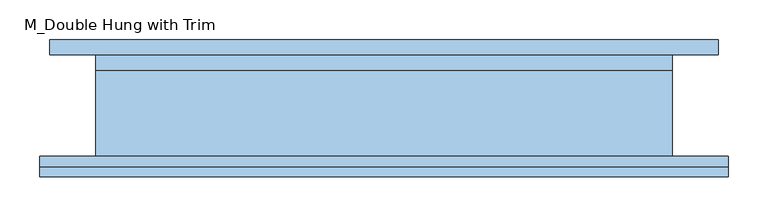
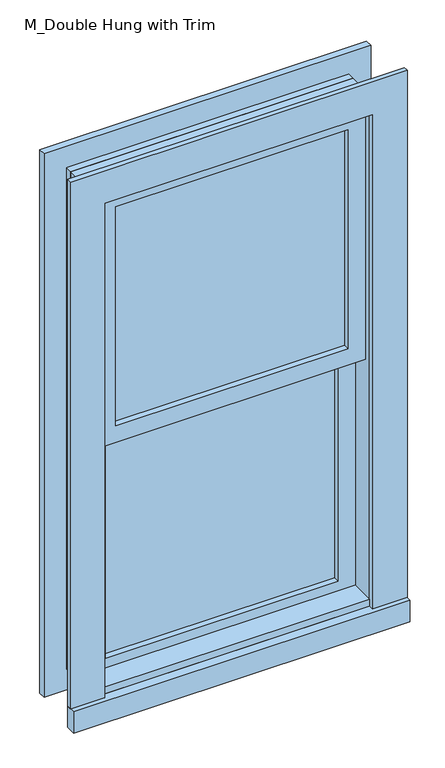
"""IFC4 building model written with IfcOpenShell, lengths in millimetres: window geometry, M_Double Hung with Trim."""

from ifc_helpers import new_model, si_unit, frame, origin, place, context, project, spatial, polyline, outline, extrude, source, transform, mapped, element, save


def m_double_hung_with_trim_c80b3b57(model_context):
    return source(origin(), model_context, "Body", "SweptSolid", [
        extrude(outline(polyline([(-298.45, 15.825), (-298.45, 28.525), (298.45, 28.525), (298.45, 15.825), (-298.45, 15.825)])), frame((0.0, 0.0, 628.65), z_axis=(0.0, 0.0, 1.0), x_axis=(1.0, 0.0, 0.0)), (0.0, 0.0, 1.0), 612.775),
        extrude(outline(polyline([(1285.875, -342.9), (584.2, -342.9), (584.2, 342.9), (1285.875, 342.9), (1285.875, -342.9)]), holes=[polyline([(1241.425, -298.45), (1241.425, 298.45), (628.65, 298.45), (628.65, -298.45), (1241.425, -298.45)])]), frame((0.0, -0.05, 0.0), z_axis=(0.0, 1.0, 0.0), x_axis=(0.0, 0.0, 1.0)), (0.0, 0.0, 1.0), 44.45),
        extrude(outline(polyline([(-431.9, -89.2), (-431.9, -63.5), (431.9, -63.5), (431.9, -89.2), (-431.9, -89.2)])), frame((0.0, 0.0, 526.95), z_axis=(0.0, 0.0, 1.0), x_axis=(1.0, 0.0, 0.0)), (0.0, 0.0, 1.0), 57.25),
        extrude(outline(polyline([(2013.05, -431.9), (526.95, -431.9), (526.95, 431.9), (2013.05, 431.9), (2013.05, -431.9)]), holes=[polyline([(1924.05, -342.9), (1924.05, 342.9), (584.2, 342.9), (584.2, -342.9), (1924.05, -342.9)])]), frame((0.0, -76.5, 0.0), z_axis=(0.0, 1.0, 0.0), x_axis=(0.0, 0.0, 1.0)), (0.0, 0.0, 1.0), 13.0),
        extrude(outline(polyline([(2000.35, 419.2), (2000.35, -419.2), (526.95, -419.2), (526.95, 419.2), (2000.35, 419.2)]), holes=[polyline([(1911.35, 330.2), (615.95, 330.2), (615.95, -330.2), (1911.35, -330.2), (1911.35, 330.2)])]), frame((0.0, 63.5, 0.0), z_axis=(0.0, 1.0, 0.0), x_axis=(0.0, 0.0, 1.0)), (0.0, 0.0, 1.0), 19.0),
        extrude(outline(polyline([(298.45, -15.925), (298.45, -28.625), (-298.45, -28.625), (-298.45, -15.925), (298.45, -15.925)])), frame((0.0, 0.0, 1285.875), z_axis=(0.0, 0.0, 1.0), x_axis=(1.0, 0.0, 0.0)), (0.0, 0.0, 1.0), 593.725),
        extrude(outline(polyline([(1924.05, -342.9), (1241.425, -342.9), (1241.425, 342.9), (1924.05, 342.9), (1924.05, -342.9)]), holes=[polyline([(1879.6, -298.45), (1879.6, 298.45), (1285.875, 298.45), (1285.875, -298.45), (1879.6, -298.45)])]), frame((0.0, -44.5, 0.0), z_axis=(0.0, 1.0, 0.0), x_axis=(0.0, 0.0, 1.0)), (0.0, 0.0, 1.0), 44.45),
        extrude(outline(polyline([(1943.1, -361.95), (584.2, -361.95), (584.2, 361.95), (1943.1, 361.95), (1943.1, -361.95)]), holes=[polyline([(1911.35, -330.2), (1911.35, 330.2), (615.95, 330.2), (615.95, -330.2), (1911.35, -330.2)])]), frame((0.0, 44.4, 0.0), z_axis=(0.0, 1.0, 0.0), x_axis=(0.0, 0.0, 1.0)), (0.0, 0.0, 1.0), 19.1),
        extrude(outline(polyline([(1943.1, 361.95), (1943.1, -361.95), (584.2, -361.95), (584.2, 361.95), (1943.1, 361.95)]), holes=[polyline([(1924.05, 342.9), (603.25, 342.9), (603.25, -342.9), (1924.05, -342.9), (1924.05, 342.9)])]), frame((0.0, -63.5, 0.0), z_axis=(0.0, 1.0, 0.0), x_axis=(0.0, 0.0, 1.0)), (0.0, 0.0, 1.0), 107.9),
    ])


if __name__ == "__main__":
    model = new_model("IFC4")
    model_context = context("Model", 3, world=origin())
    ifc_project = project(units=[si_unit("LENGTHUNIT", "METRE", prefix="MILLI")], contexts=[model_context])
    site = spatial("IfcSite", under=ifc_project)
    building = spatial("IfcBuilding", under=site)
    placement = place(None, origin())
    m_double_hung_with_trim_shape = m_double_hung_with_trim_c80b3b57(model_context)
    element("IfcWindow", 1, ObjectType="M_Double Hung with Trim : 57\" x 54\" @ 23\" b", at=placement, inside=building, context=model_context, shape_type="MappedRepresentation", body=[
        mapped(m_double_hung_with_trim_shape, transform((0.0, 0.0, 0.0), x_axis=(1.0, 0.0, 0.0), y_axis=(0.0, 1.0, 0.0), z_axis=(0.0, 0.0, 1.0))),
    ])
    save(model, "model.ifc")

# Revit data of these elements
# Type "M_Double Hung with Trim : 57\" x 54\" @ 23\" b"
#   Type Mark = "63"
#   Construction Type Id = "GSP4R"
#   Analytic Construction = "1/8 in Pilkington single glazing"
#   Visual Light Transmittance = 0.9
#   Thermal Resistance (R) = 0.271106 (m²·K)/W
#   Solar Heat Gain Coefficient = 0.78
#   Heat Transfer Coefficient (U) = 3.6886 W/(m²·K)
#   Height = 4' - 5 1/2"
#   Default Sill Height = 1' - 11"
#   Trim Projection - Ext. = 0' - 0.51181"
#   Trim Projection - Int. = 0' - 0.74803"
#   Trim Width - Exterior = 0' - 3.50394"
#   Trim Width - Interior = 0' - 3.50394"
#   Width = 2' - 4 1/2"
#   Window Inset = 0' - 0.74803"
#   Glass Pane Material = EXISTING WINDOW
#   Sash = Trim
#   Trim Exterior Material = Trim
#   Trim Interior Material = Trim
#   Wall Closure = (empty or 0)
# Element 1 (IfcWindow, "M_Double Hung with Trim : 57\" x 54\" @ 23\" b")
#   Materials on its faces: "Trim", "EXISTING WINDOW"
# Materials
#   "EXISTING WINDOW": class "Glass", colour RGB 218 227 224, transparency 0.85, Description = "Soda Lime Glass", Cost = 0
#   "Trim": class "Wood", colour RGB 250 251 245, transparency 0, Cost = 0
